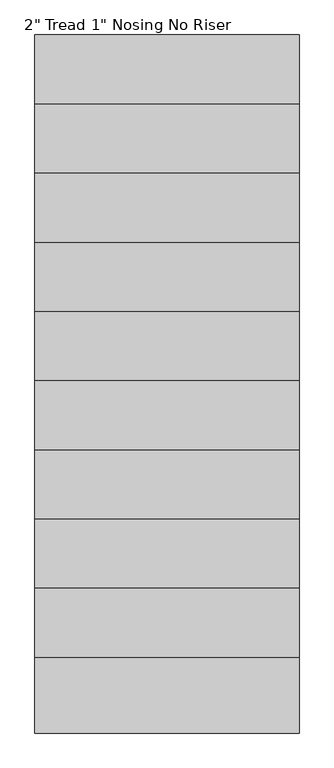
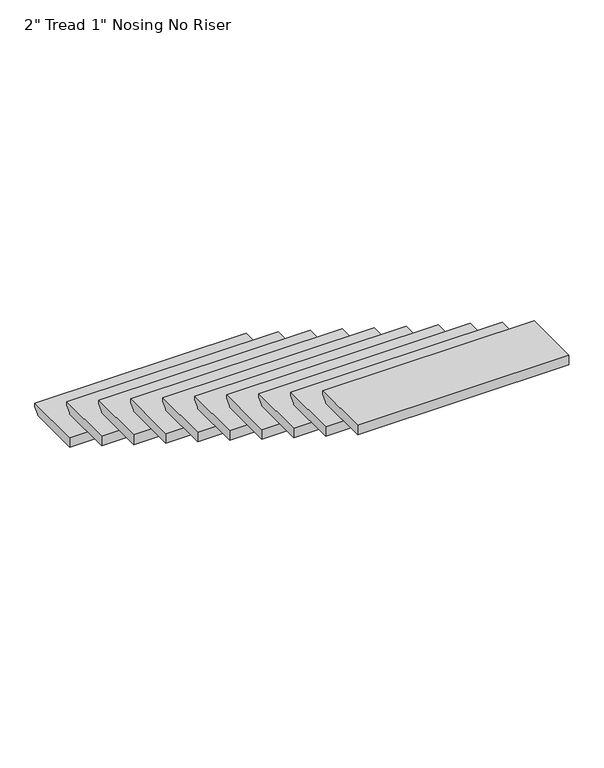
"""IFC4 building model written with IfcOpenShell, lengths in millimetres: stair flight geometry."""

import ifcopenshell
import ifcopenshell.guid

model = None  # the IFC model being written
_history = None  # IfcOwnerHistory: only IFC2X3 demands one
_inside = {}  # id of a spatial element -> (the spatial element, [elements in it])
_under = {}  # id of a project, library or spatial element -> (it, [spatial elements below it])
_declared = {}  # id of a project -> (the project, [libraries it declares])
_typed = {}  # id of a type object -> (the type object, [elements of that type])
_made_of = {}  # id of a material, layer set ... -> (it, [elements and type objects made of it])


def new_model(schema):
    """Start an empty IFC model of exactly this schema.

    Asked for "IFC4X3", IfcOpenShell would pick the latest addendum, in which some entities
    have other attributes; the version numbers below select the first issue.
    IFC2X3 requires an IfcOwnerHistory on every rooted entity: one is made here for all.
    """
    global model, _history
    if schema == "IFC4X3":
        model = ifcopenshell.file(schema_version=(4, 3, 0, 0))
    else:
        model = ifcopenshell.file(schema=schema)
    _inside.clear()
    _under.clear()
    _declared.clear()
    _typed.clear()
    _made_of.clear()
    _history = None
    if model.schema == "IFC2X3":
        org = make("IfcOrganization", Name="unknown")
        user = make(
            "IfcPersonAndOrganization",
            ThePerson=make("IfcPerson", FamilyName="unknown"),
            TheOrganization=org,
        )
        app = make(
            "IfcApplication",
            ApplicationDeveloper=org,
            Version="unknown",
            ApplicationFullName="unknown",
            ApplicationIdentifier="unknown",
        )
        _history = make(
            "IfcOwnerHistory",
            OwningUser=user,
            OwningApplication=app,
            ChangeAction="ADDED",
            CreationDate=0,
        )
    return model


def make(cls, **values):
    """One entity of the class cls with the attributes given. An attribute that is None is left unset."""
    return model.create_entity(
        cls, **{name: value for name, value in values.items() if value is not None}
    )


def rooted(cls, **values):
    """An entity with a GlobalId (a new one), such as an element, a storey or a relation."""
    return make(cls, GlobalId=ifcopenshell.guid.new(), OwnerHistory=_history, **values)


def si_unit(unit_type, name, prefix=None):
    """IfcSIUnit, for example si_unit("LENGTHUNIT", "METRE", prefix="MILLI")."""
    return make("IfcSIUnit", UnitType=unit_type, Prefix=prefix, Name=name)


def assignment(units):
    """IfcUnitAssignment: the units of a project."""
    return None if units is None else make("IfcUnitAssignment", Units=units)


def point(xyz):
    """IfcCartesianPoint."""
    return None if xyz is None else make("IfcCartesianPoint", Coordinates=xyz)


def direction(xyz):
    """IfcDirection."""
    return None if xyz is None else make("IfcDirection", DirectionRatios=xyz)


def frame(location, z_axis=None, x_axis=None):
    """IfcAxis2Placement3D, a coordinate frame: its origin and axes. An axis left out is left unset."""
    return make(
        "IfcAxis2Placement3D",
        Location=point(location),
        Axis=direction(z_axis),
        RefDirection=direction(x_axis),
    )


def origin():
    """The frame at (0, 0, 0) with its axes left unset."""
    return frame((0.0, 0.0, 0.0))


def place(relative_to, where):
    """IfcLocalPlacement: puts the frame where relative to a parent placement (None: the world)."""
    return make(
        "IfcLocalPlacement", PlacementRelTo=relative_to, RelativePlacement=where
    )


def context(
    kind, dimensions, precision=None, world=None, true_north=None, identifier=None
):
    """IfcGeometricRepresentationContext, for example the 3D "Model" context."""
    return make(
        "IfcGeometricRepresentationContext",
        ContextIdentifier=identifier,
        ContextType=kind,
        CoordinateSpaceDimension=dimensions,
        Precision=precision,
        WorldCoordinateSystem=world,
        TrueNorth=true_north,
    )


def project(units=None, contexts=None):
    """IfcProject with its units and contexts."""
    return rooted(
        "IfcProject",
        Name="project",
        RepresentationContexts=contexts,
        UnitsInContext=assignment(units),
    )


def spatial(cls, under=None, at=None, **own):
    """A site, building, storey or space (cls), placed at a placement, below another one or the project."""
    s = rooted(cls, ObjectPlacement=at, **own)
    if under is not None:
        _under.setdefault(under.id(), (under, []))[1].append(s)
    return s


def polyline(points):
    """IfcPolyline through the points."""
    return make("IfcPolyline", Points=[point(p) for p in points])


def outline(outer, holes=None, kind="AREA"):
    """IfcArbitraryClosedProfileDef: a profile drawn as a closed curve; with holes, ...WithVoids."""
    if holes is None:
        return make("IfcArbitraryClosedProfileDef", ProfileType=kind, OuterCurve=outer)
    return make(
        "IfcArbitraryProfileDefWithVoids",
        ProfileType=kind,
        OuterCurve=outer,
        InnerCurves=holes,
    )


def extrude(swept, where, along, depth):
    """IfcExtrudedAreaSolid: the profile swept, set in the frame where, extruded along a direction by depth."""
    return make(
        "IfcExtrudedAreaSolid",
        SweptArea=swept,
        Position=where,
        ExtrudedDirection=direction(along),
        Depth=depth,
    )


def shape(context_of_items, identifier, shape_type, items):
    """IfcShapeRepresentation: the items that make up one representation, for example the "Body"."""
    return make(
        "IfcShapeRepresentation",
        ContextOfItems=context_of_items,
        RepresentationIdentifier=identifier,
        RepresentationType=shape_type,
        Items=items,
    )


def source(mapping_origin, context_of_items, identifier, shape_type, items):
    """IfcRepresentationMap: a shape defined once, which mapped items show again and again."""
    return make(
        "IfcRepresentationMap",
        MappingOrigin=mapping_origin,
        MappedRepresentation=shape(context_of_items, identifier, shape_type, items),
    )


def transform(
    local_origin,
    x_axis=None,
    y_axis=None,
    z_axis=None,
    scale=None,
    scale2=None,
    scale3=None,
    uniform=True,
):
    """IfcCartesianTransformationOperator3D, or its non-uniform kind. x_axis, y_axis, z_axis: its Axis1, 2, 3."""
    if uniform:
        return make(
            "IfcCartesianTransformationOperator3D",
            Axis1=direction(x_axis),
            Axis2=direction(y_axis),
            LocalOrigin=point(local_origin),
            Scale=scale,
            Axis3=direction(z_axis),
        )
    return make(
        "IfcCartesianTransformationOperator3DnonUniform",
        Axis1=direction(x_axis),
        Axis2=direction(y_axis),
        LocalOrigin=point(local_origin),
        Scale=scale,
        Axis3=direction(z_axis),
        Scale2=scale2,
        Scale3=scale3,
    )


def mapped(mapping_source, mapping_target):
    """IfcMappedItem: shows the shape of a source again, moved by a transform."""
    return make(
        "IfcMappedItem", MappingSource=mapping_source, MappingTarget=mapping_target
    )


def made_of(thing, what):
    """Note that an element or type object is made of a material, layer set ...; save() writes the relation."""
    if what is not None:
        _made_of.setdefault(what.id(), (what, []))[1].append(thing)
    return thing


def element(
    cls,
    number,
    at=None,
    inside=None,
    cuts=None,
    type_object=None,
    material=None,
    context=None,
    identifier="Body",
    shape_type=None,
    held_by="IfcProductDefinitionShape",
    body=None,
    shapes=None,
    **own,
):
    """One element of the class cls, such as IfcWall. Its Tag is "e" and its number.

    at: its placement. inside: the storey or other place that contains it. cuts: it is an
    opening in that element (IfcRelVoidsElement). A single representation is given by context,
    identifier, shape_type and body (its items); several are given by shapes. held_by: the class
    of the entity that holds the representations. save() writes the other relations.
    """
    e = rooted(cls, Tag="e%d" % number, ObjectPlacement=at, **own)
    if body is not None:
        shapes = [shape(context, identifier, shape_type, body)]
    if shapes is not None:
        e.Representation = make(held_by, Representations=shapes)
    if inside is not None:
        _inside.setdefault(inside.id(), (inside, []))[1].append(e)
    if cuts is not None:
        rooted(
            "IfcRelVoidsElement", RelatingBuildingElement=cuts, RelatedOpeningElement=e
        )
    if type_object is not None:
        _typed.setdefault(type_object.id(), (type_object, []))[1].append(e)
    return made_of(e, material)


def aggregate(whole, parts):
    """IfcRelAggregates: a whole, such as a stair, and the parts it consists of."""
    return rooted("IfcRelAggregates", RelatingObject=whole, RelatedObjects=parts)


def save(model, path):
    """Write the relations noted so far, then the file.

    IfcRelAggregates (storeys below a building ...), IfcRelContainedInSpatialStructure (elements
    in a storey), IfcRelDefinesByType, IfcRelAssociatesMaterial and IfcRelDeclares: one each for
    every whole, place, type object, material and project.
    """
    for whole, parts in _under.values():
        aggregate(whole, parts)
    for where, things in _inside.values():
        rooted(
            "IfcRelContainedInSpatialStructure",
            RelatedElements=things,
            RelatingStructure=where,
        )
    for kind, things in _typed.values():
        rooted("IfcRelDefinesByType", RelatedObjects=things, RelatingType=kind)
    for what, things in _made_of.values():
        rooted("IfcRelAssociatesMaterial", RelatedObjects=things, RelatingMaterial=what)
    for by, libraries in _declared.values():
        rooted("IfcRelDeclares", RelatingContext=by, RelatedDefinitions=libraries)
    model.write(path)


def stair_flight_61c66307(model_context):
    return source(origin(), model_context, "Body", "SweptSolid", [
        extrude(outline(polyline([(613.7695005, 32777.0434783), (918.5695005, 32777.0434783), (918.5695005, 32757.9934783), (893.1695005, 32732.5934783), (893.1695005, 32726.2434783), (613.7695005, 32726.2434783), (613.7695005, 32777.0434783)])), frame((-10143.1704607, 0.0, 0.0), z_axis=(1.0, 0.0, 0.0), x_axis=(0.0, 1.0, 0.0)), (0.0, 0.0, 1.0), 1066.8),
        extrude(outline(polyline([(334.3695005, 32953.7391304), (639.1695005, 32953.7391304), (639.1695005, 32934.6891304), (613.7695005, 32909.2891304), (613.7695005, 32902.9391304), (334.3695005, 32902.9391304), (334.3695005, 32953.7391304)])), frame((-10143.1704607, 0.0, 0.0), z_axis=(1.0, 0.0, 0.0), x_axis=(0.0, 1.0, 0.0)), (0.0, 0.0, 1.0), 1066.8),
        extrude(outline(polyline([(54.9695005, 33130.4347826), (359.7695005, 33130.4347826), (359.7695005, 33111.3847826), (334.3695005, 33085.9847826), (334.3695005, 33079.6347826), (54.9695005, 33079.6347826), (54.9695005, 33130.4347826)])), frame((-10143.1704607, 0.0, 0.0), z_axis=(1.0, 0.0, 0.0), x_axis=(0.0, 1.0, 0.0)), (0.0, 0.0, 1.0), 1066.8),
        extrude(outline(polyline([(-224.4304995, 33307.1304348), (80.3695005, 33307.1304348), (80.3695005, 33288.0804348), (54.9695005, 33262.6804348), (54.9695005, 33256.3304348), (-224.4304995, 33256.3304348), (-224.4304995, 33307.1304348)])), frame((-10143.1704607, 0.0, 0.0), z_axis=(1.0, 0.0, 0.0), x_axis=(0.0, 1.0, 0.0)), (0.0, 0.0, 1.0), 1066.8),
        extrude(outline(polyline([(-503.8304995, 33483.826087), (-199.0304995, 33483.826087), (-199.0304995, 33464.776087), (-224.4304995, 33439.376087), (-224.4304995, 33433.026087), (-503.8304995, 33433.026087), (-503.8304995, 33483.826087)])), frame((-10143.1704607, 0.0, 0.0), z_axis=(1.0, 0.0, 0.0), x_axis=(0.0, 1.0, 0.0)), (0.0, 0.0, 1.0), 1066.8),
        extrude(outline(polyline([(-783.2304995, 33660.5217391), (-478.4304995, 33660.5217391), (-478.4304995, 33641.4717391), (-503.8304995, 33616.0717391), (-503.8304995, 33609.7217391), (-783.2304995, 33609.7217391), (-783.2304995, 33660.5217391)])), frame((-10143.1704607, 0.0, 0.0), z_axis=(1.0, 0.0, 0.0), x_axis=(0.0, 1.0, 0.0)), (0.0, 0.0, 1.0), 1066.8),
        extrude(outline(polyline([(-1062.6304995, 33837.2173913), (-757.8304995, 33837.2173913), (-757.8304995, 33818.1673913), (-783.2304995, 33792.7673913), (-783.2304995, 33786.4173913), (-1062.6304995, 33786.4173913), (-1062.6304995, 33837.2173913)])), frame((-10143.1704607, 0.0, 0.0), z_axis=(1.0, 0.0, 0.0), x_axis=(0.0, 1.0, 0.0)), (0.0, 0.0, 1.0), 1066.8),
        extrude(outline(polyline([(-1342.0304995, 34013.9130435), (-1037.2304995, 34013.9130435), (-1037.2304995, 33994.8630435), (-1062.6304995, 33969.4630435), (-1062.6304995, 33963.1130435), (-1342.0304995, 33963.1130435), (-1342.0304995, 34013.9130435)])), frame((-10143.1704607, 0.0, 0.0), z_axis=(1.0, 0.0, 0.0), x_axis=(0.0, 1.0, 0.0)), (0.0, 0.0, 1.0), 1066.8),
        extrude(outline(polyline([(-1621.4304995, 34190.6086957), (-1316.6304995, 34190.6086957), (-1316.6304995, 34171.5586957), (-1342.0304995, 34146.1586957), (-1342.0304995, 34139.8086957), (-1621.4304995, 34139.8086957), (-1621.4304995, 34190.6086957)])), frame((-10143.1704607, 0.0, 0.0), z_axis=(1.0, 0.0, 0.0), x_axis=(0.0, 1.0, 0.0)), (0.0, 0.0, 1.0), 1066.8),
        extrude(outline(polyline([(-1900.8304995, 34367.3043478), (-1596.0304995, 34367.3043478), (-1596.0304995, 34348.2543478), (-1621.4304995, 34322.8543478), (-1621.4304995, 34316.5043478), (-1900.8304995, 34316.5043478), (-1900.8304995, 34367.3043478)])), frame((-10143.1704607, 0.0, 0.0), z_axis=(1.0, 0.0, 0.0), x_axis=(0.0, 1.0, 0.0)), (0.0, 0.0, 1.0), 1066.8),
    ])


if __name__ == "__main__":
    model = new_model("IFC4")
    model_context = context("Model", 3, world=origin())
    ifc_project = project(units=[si_unit("LENGTHUNIT", "METRE", prefix="MILLI")], contexts=[model_context])
    site = spatial("IfcSite", under=ifc_project)
    building = spatial("IfcBuilding", under=site)
    placement = place(None, origin())
    stair_flight_shape = stair_flight_61c66307(model_context)
    element("IfcStairFlight", 1, ObjectType="2\" Tread 1\" Nosing No Riser", at=placement, inside=building, context=model_context, shape_type="MappedRepresentation", body=[
        mapped(stair_flight_shape, transform((0.0, 0.0, 0.0), x_axis=(1.0, 0.0, 0.0), y_axis=(0.0, 1.0, 0.0), z_axis=(0.0, 0.0, 1.0))),
    ])
    save(model, "model.ifc")
